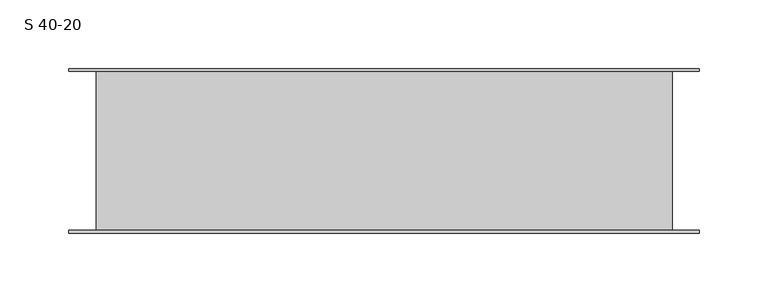
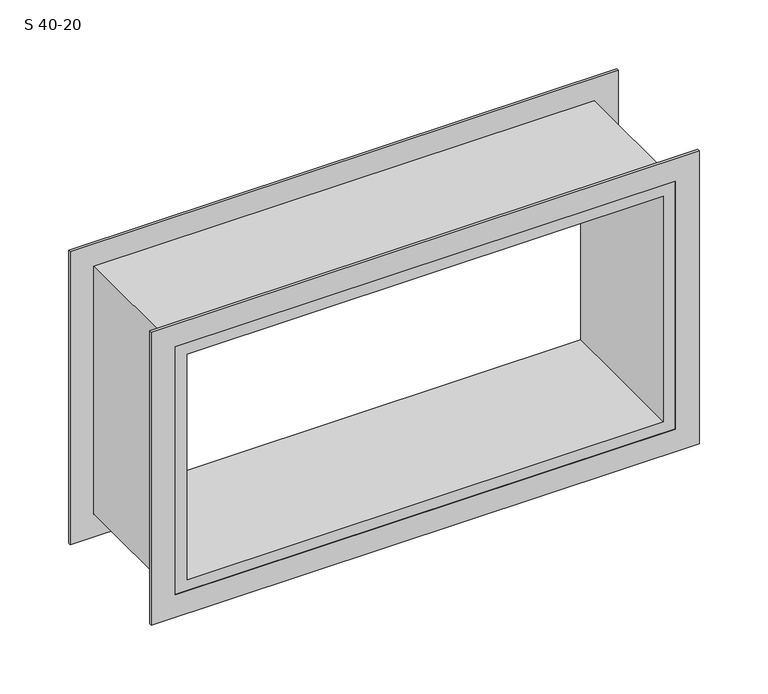
"""IFC4 building model written with IfcOpenShell, lengths in millimetres: proxy geometry, Регулирующая заслонка S : S 40-20."""

import ifcopenshell
import ifcopenshell.guid

model = None  # the IFC model being written
_history = None  # IfcOwnerHistory: only IFC2X3 demands one
_inside = {}  # id of a spatial element -> (the spatial element, [elements in it])
_under = {}  # id of a project, library or spatial element -> (it, [spatial elements below it])
_declared = {}  # id of a project -> (the project, [libraries it declares])
_typed = {}  # id of a type object -> (the type object, [elements of that type])
_made_of = {}  # id of a material, layer set ... -> (it, [elements and type objects made of it])


def new_model(schema):
    """Start an empty IFC model of exactly this schema.

    Asked for "IFC4X3", IfcOpenShell would pick the latest addendum, in which some entities
    have other attributes; the version numbers below select the first issue.
    IFC2X3 requires an IfcOwnerHistory on every rooted entity: one is made here for all.
    """
    global model, _history
    if schema == "IFC4X3":
        model = ifcopenshell.file(schema_version=(4, 3, 0, 0))
    else:
        model = ifcopenshell.file(schema=schema)
    _inside.clear()
    _under.clear()
    _declared.clear()
    _typed.clear()
    _made_of.clear()
    _history = None
    if model.schema == "IFC2X3":
        org = make("IfcOrganization", Name="unknown")
        user = make(
            "IfcPersonAndOrganization",
            ThePerson=make("IfcPerson", FamilyName="unknown"),
            TheOrganization=org,
        )
        app = make(
            "IfcApplication",
            ApplicationDeveloper=org,
            Version="unknown",
            ApplicationFullName="unknown",
            ApplicationIdentifier="unknown",
        )
        _history = make(
            "IfcOwnerHistory",
            OwningUser=user,
            OwningApplication=app,
            ChangeAction="ADDED",
            CreationDate=0,
        )
    return model


def make(cls, **values):
    """One entity of the class cls with the attributes given. An attribute that is None is left unset."""
    return model.create_entity(
        cls, **{name: value for name, value in values.items() if value is not None}
    )


def rooted(cls, **values):
    """An entity with a GlobalId (a new one), such as an element, a storey or a relation."""
    return make(cls, GlobalId=ifcopenshell.guid.new(), OwnerHistory=_history, **values)


def si_unit(unit_type, name, prefix=None):
    """IfcSIUnit, for example si_unit("LENGTHUNIT", "METRE", prefix="MILLI")."""
    return make("IfcSIUnit", UnitType=unit_type, Prefix=prefix, Name=name)


def assignment(units):
    """IfcUnitAssignment: the units of a project."""
    return None if units is None else make("IfcUnitAssignment", Units=units)


def point(xyz):
    """IfcCartesianPoint."""
    return None if xyz is None else make("IfcCartesianPoint", Coordinates=xyz)


def direction(xyz):
    """IfcDirection."""
    return None if xyz is None else make("IfcDirection", DirectionRatios=xyz)


def frame(location, z_axis=None, x_axis=None):
    """IfcAxis2Placement3D, a coordinate frame: its origin and axes. An axis left out is left unset."""
    return make(
        "IfcAxis2Placement3D",
        Location=point(location),
        Axis=direction(z_axis),
        RefDirection=direction(x_axis),
    )


def origin():
    """The frame at (0, 0, 0) with its axes left unset."""
    return frame((0.0, 0.0, 0.0))


def place(relative_to, where):
    """IfcLocalPlacement: puts the frame where relative to a parent placement (None: the world)."""
    return make(
        "IfcLocalPlacement", PlacementRelTo=relative_to, RelativePlacement=where
    )


def context(
    kind, dimensions, precision=None, world=None, true_north=None, identifier=None
):
    """IfcGeometricRepresentationContext, for example the 3D "Model" context."""
    return make(
        "IfcGeometricRepresentationContext",
        ContextIdentifier=identifier,
        ContextType=kind,
        CoordinateSpaceDimension=dimensions,
        Precision=precision,
        WorldCoordinateSystem=world,
        TrueNorth=true_north,
    )


def project(units=None, contexts=None):
    """IfcProject with its units and contexts."""
    return rooted(
        "IfcProject",
        Name="project",
        RepresentationContexts=contexts,
        UnitsInContext=assignment(units),
    )


def spatial(cls, under=None, at=None, **own):
    """A site, building, storey or space (cls), placed at a placement, below another one or the project."""
    s = rooted(cls, ObjectPlacement=at, **own)
    if under is not None:
        _under.setdefault(under.id(), (under, []))[1].append(s)
    return s


def polyline(points):
    """IfcPolyline through the points."""
    return make("IfcPolyline", Points=[point(p) for p in points])


def outline(outer, holes=None, kind="AREA"):
    """IfcArbitraryClosedProfileDef: a profile drawn as a closed curve; with holes, ...WithVoids."""
    if holes is None:
        return make("IfcArbitraryClosedProfileDef", ProfileType=kind, OuterCurve=outer)
    return make(
        "IfcArbitraryProfileDefWithVoids",
        ProfileType=kind,
        OuterCurve=outer,
        InnerCurves=holes,
    )


def extrude(swept, where, along, depth):
    """IfcExtrudedAreaSolid: the profile swept, set in the frame where, extruded along a direction by depth."""
    return make(
        "IfcExtrudedAreaSolid",
        SweptArea=swept,
        Position=where,
        ExtrudedDirection=direction(along),
        Depth=depth,
    )


def shape(context_of_items, identifier, shape_type, items):
    """IfcShapeRepresentation: the items that make up one representation, for example the "Body"."""
    return make(
        "IfcShapeRepresentation",
        ContextOfItems=context_of_items,
        RepresentationIdentifier=identifier,
        RepresentationType=shape_type,
        Items=items,
    )


def source(mapping_origin, context_of_items, identifier, shape_type, items):
    """IfcRepresentationMap: a shape defined once, which mapped items show again and again."""
    return make(
        "IfcRepresentationMap",
        MappingOrigin=mapping_origin,
        MappedRepresentation=shape(context_of_items, identifier, shape_type, items),
    )


def transform(
    local_origin,
    x_axis=None,
    y_axis=None,
    z_axis=None,
    scale=None,
    scale2=None,
    scale3=None,
    uniform=True,
):
    """IfcCartesianTransformationOperator3D, or its non-uniform kind. x_axis, y_axis, z_axis: its Axis1, 2, 3."""
    if uniform:
        return make(
            "IfcCartesianTransformationOperator3D",
            Axis1=direction(x_axis),
            Axis2=direction(y_axis),
            LocalOrigin=point(local_origin),
            Scale=scale,
            Axis3=direction(z_axis),
        )
    return make(
        "IfcCartesianTransformationOperator3DnonUniform",
        Axis1=direction(x_axis),
        Axis2=direction(y_axis),
        LocalOrigin=point(local_origin),
        Scale=scale,
        Axis3=direction(z_axis),
        Scale2=scale2,
        Scale3=scale3,
    )


def mapped(mapping_source, mapping_target):
    """IfcMappedItem: shows the shape of a source again, moved by a transform."""
    return make(
        "IfcMappedItem", MappingSource=mapping_source, MappingTarget=mapping_target
    )


def made_of(thing, what):
    """Note that an element or type object is made of a material, layer set ...; save() writes the relation."""
    if what is not None:
        _made_of.setdefault(what.id(), (what, []))[1].append(thing)
    return thing


def element(
    cls,
    number,
    at=None,
    inside=None,
    cuts=None,
    type_object=None,
    material=None,
    context=None,
    identifier="Body",
    shape_type=None,
    held_by="IfcProductDefinitionShape",
    body=None,
    shapes=None,
    **own,
):
    """One element of the class cls, such as IfcWall. Its Tag is "e" and its number.

    at: its placement. inside: the storey or other place that contains it. cuts: it is an
    opening in that element (IfcRelVoidsElement). A single representation is given by context,
    identifier, shape_type and body (its items); several are given by shapes. held_by: the class
    of the entity that holds the representations. save() writes the other relations.
    """
    e = rooted(cls, Tag="e%d" % number, ObjectPlacement=at, **own)
    if body is not None:
        shapes = [shape(context, identifier, shape_type, body)]
    if shapes is not None:
        e.Representation = make(held_by, Representations=shapes)
    if inside is not None:
        _inside.setdefault(inside.id(), (inside, []))[1].append(e)
    if cuts is not None:
        rooted(
            "IfcRelVoidsElement", RelatingBuildingElement=cuts, RelatedOpeningElement=e
        )
    if type_object is not None:
        _typed.setdefault(type_object.id(), (type_object, []))[1].append(e)
    return made_of(e, material)


def aggregate(whole, parts):
    """IfcRelAggregates: a whole, such as a stair, and the parts it consists of."""
    return rooted("IfcRelAggregates", RelatingObject=whole, RelatedObjects=parts)


def save(model, path):
    """Write the relations noted so far, then the file.

    IfcRelAggregates (storeys below a building ...), IfcRelContainedInSpatialStructure (elements
    in a storey), IfcRelDefinesByType, IfcRelAssociatesMaterial and IfcRelDeclares: one each for
    every whole, place, type object, material and project.
    """
    for whole, parts in _under.values():
        aggregate(whole, parts)
    for where, things in _inside.values():
        rooted(
            "IfcRelContainedInSpatialStructure",
            RelatedElements=things,
            RelatingStructure=where,
        )
    for kind, things in _typed.values():
        rooted("IfcRelDefinesByType", RelatedObjects=things, RelatingType=kind)
    for what, things in _made_of.values():
        rooted("IfcRelAssociatesMaterial", RelatedObjects=things, RelatingMaterial=what)
    for by, libraries in _declared.values():
        rooted("IfcRelDeclares", RelatingContext=by, RelatedDefinitions=libraries)
    model.write(path)


def s_40_20_78d282e4(model_context):
    return source(origin(), model_context, "Body", "SweptSolid", [
        extrude(outline(polyline([(130.0, 230.0), (130.0, -230.0), (-130.0, -230.0), (-130.0, 230.0), (130.0, 230.0)]), holes=[polyline([(-110.0, 210.0), (-110.0, -210.0), (110.0, -210.0), (110.0, 210.0), (-110.0, 210.0)])]), frame((0.0, 58.0, 0.0), z_axis=(0.0, 1.0, 0.0), x_axis=(0.0, 0.0, 1.0)), (0.0, 0.0, 1.0), 2.0),
        extrude(outline(polyline([(130.0, -230.0), (-130.0, -230.0), (-130.0, 230.0), (130.0, 230.0), (130.0, -230.0)]), holes=[polyline([(110.0, 210.0), (-110.0, 210.0), (-110.0, -210.0), (110.0, -210.0), (110.0, 210.0)])]), frame((0.0, -60.0, 0.0), z_axis=(0.0, 1.0, 0.0), x_axis=(0.0, 0.0, 1.0)), (0.0, 0.0, 1.0), 2.0),
        extrude(outline(polyline([(110.0, 210.0), (110.0, -210.0), (-110.0, -210.0), (-110.0, 210.0), (110.0, 210.0)]), holes=[polyline([(100.0, 200.0), (-100.0, 200.0), (-100.0, -200.0), (100.0, -200.0), (100.0, 200.0)])]), frame((0.0, -60.0, 0.0), z_axis=(0.0, 1.0, 0.0), x_axis=(0.0, 0.0, 1.0)), (0.0, 0.0, 1.0), 120.0),
    ])


if __name__ == "__main__":
    model = new_model("IFC4")
    model_context = context("Model", 3, world=origin())
    ifc_project = project(units=[si_unit("LENGTHUNIT", "METRE", prefix="MILLI")], contexts=[model_context])
    site = spatial("IfcSite", under=ifc_project)
    building = spatial("IfcBuilding", under=site)
    placement = place(None, origin())
    s_40_20_shape = s_40_20_78d282e4(model_context)
    element("IfcBuildingElementProxy", 1, Name="Регулирующая заслонка S : S 40-20", ObjectType="Регулирующая заслонка S : S 40-20", at=placement, inside=building, context=model_context, shape_type="MappedRepresentation", body=[
        mapped(s_40_20_shape, transform((0.0, 0.0, 0.0), x_axis=(1.0, 0.0, 0.0), y_axis=(0.0, 1.0, 0.0), z_axis=(0.0, 0.0, 1.0))),
    ])
    save(model, "model.ifc")

# Revit data of these elements
# Type "Регулирующая заслонка S : S 40-20"
#   Manufacturer = "WAER"
#   URL = "https://waer-air.com/"
#   ADSK_Система_Имя [instance default] = ""
#   ADSK_Наименование краткое = "S 40-20"
#   ADSK_Наименование = "Регулирующая заслонка S 40-20"
#   ADSK_Масса_Текст = "3.6"
#   ADSK_Марка = ""
#   ADSK_Код изделия = ""
#   ADSK_Завод-изготовитель = "WAER"
#   ADSK_Единица измерения = "шт."
#   ширина = 400 mm
#   толщина = 10 mm
#   высота = 200 mm
#   ADSK_Расход воздуха = 0 m³/h
#   ADSK_Размер_Ширина = 420 mm
#   ADSK_Размер_Высота = 220 mm
#   ADSK_Потеря давления воздуха = 0.0 Pa
#   ADSK_Масса = 3.6
#   ADSK_Количество = 1
#   Default Elevation = 0
#   Keynote = ""
